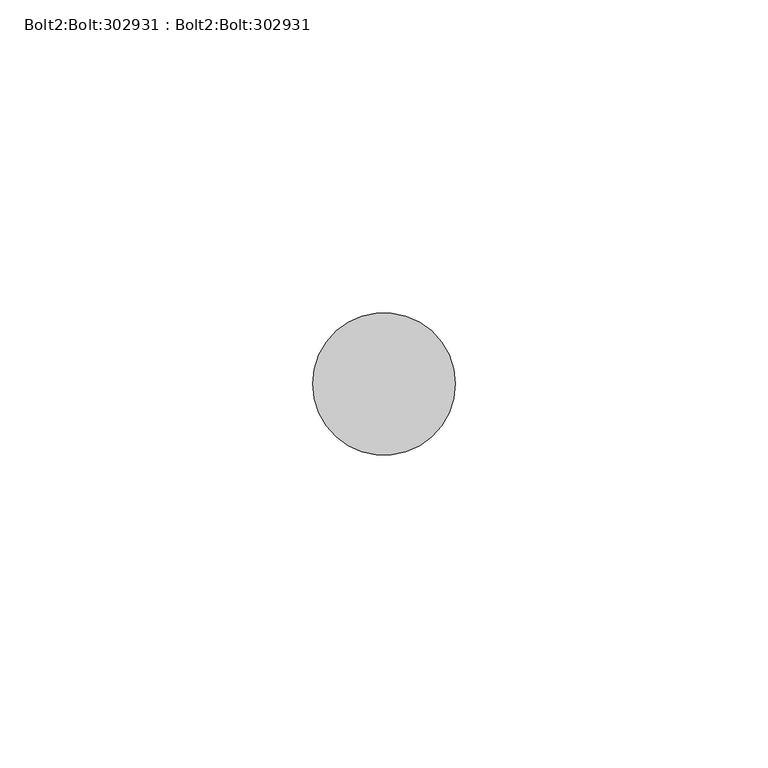
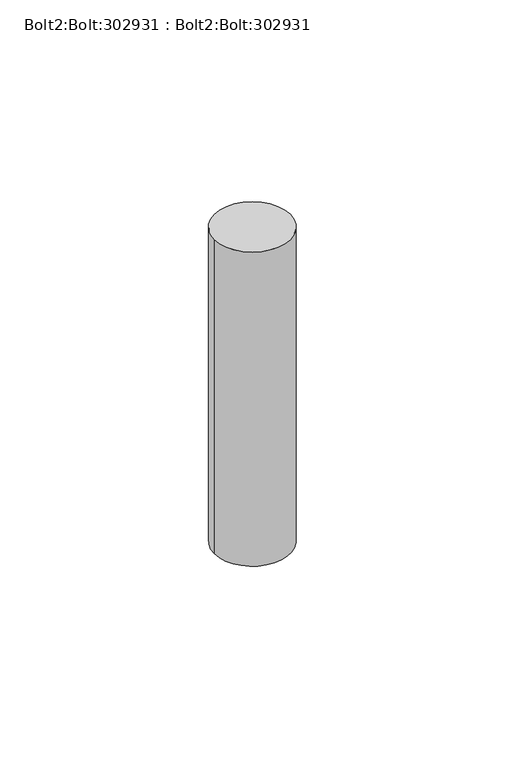
"""IFC4 building model written with IfcOpenShell, lengths in millimetres: proxy geometry, Bolt2:Bolt:302931 : Bolt2:Bolt:302931."""

from ifc_helpers import new_model, si_unit, point, frame, frame_2d, origin, place, context, project, spatial, circle_curve, trimmed, segment, composite_curve, outline, extrude, source, transform, mapped, element, save


def bolt2_bolt_302931_bolt2_bolt_302931_9da7799a(model_context):
    return source(origin(), model_context, "Body", "SweptSolid", [
        extrude(outline(composite_curve([segment(trimmed(circle_curve(frame_2d((12028.9793228, -1503.5124296)), 11.4045168), [point((12017.574806, -1503.5124296))], [point((12040.3838396, -1503.5124296))], False, "CARTESIAN"), True, "CONTINUOUS"), segment(trimmed(circle_curve(frame_2d((12028.9793228, -1503.5124296)), 11.4045168), [point((12040.3838396, -1503.5124296))], [point((12017.574806, -1503.5124296))], False, "CARTESIAN"), True, "CONTINUOUS")], self_intersect=False)), frame((0.0, 0.0, 39994.0914664), z_axis=(0.0, 0.0, 1.0), x_axis=(1.0, 0.0, 0.0)), (0.0, 0.0, 1.0), 99.5545336),
    ])


if __name__ == "__main__":
    model = new_model("IFC4")
    model_context = context("Model", 3, world=origin())
    ifc_project = project(units=[si_unit("LENGTHUNIT", "METRE", prefix="MILLI")], contexts=[model_context])
    site = spatial("IfcSite", under=ifc_project)
    building = spatial("IfcBuilding", under=site)
    placement = place(None, origin())
    bolt2_bolt_302931_bolt2_bolt_302931_shape = bolt2_bolt_302931_bolt2_bolt_302931_9da7799a(model_context)
    element("IfcBuildingElementProxy", 1, Name="Bolt2:Bolt:302931 : Bolt2:Bolt:302931", ObjectType="Bolt2:Bolt:302931 : Bolt2:Bolt:302931", at=placement, inside=building, context=model_context, shape_type="MappedRepresentation", body=[
        mapped(bolt2_bolt_302931_bolt2_bolt_302931_shape, transform((0.0, 0.0, 0.0), x_axis=(1.0, 0.0, 0.0), y_axis=(0.0, 1.0, 0.0), z_axis=(0.0, 0.0, 1.0))),
    ])
    save(model, "model.ifc")

# Revit data of these elements
# Type "Bolt2:Bolt:302931 : Bolt2:Bolt:302931"
#   NameOverride = "Bolt2:Bolt:302931"
#   ObjectTypeOverride = "Bolt2:Bolt"
#   Reference = "Bolt"
#   Category = "Generic Models"
#   Tag = "302931"
# Element 1 (IfcBuildingElementProxy, "Bolt2:Bolt:302931 : Bolt2:Bolt:302931")
#   Materials on its faces: "BOLTS CONCEALED BY FLOOR FINISH"
# Materials
#   "BOLTS CONCEALED BY FLOOR FINISH": class "Unassigned", colour RGB 128 128 128, transparency 0
